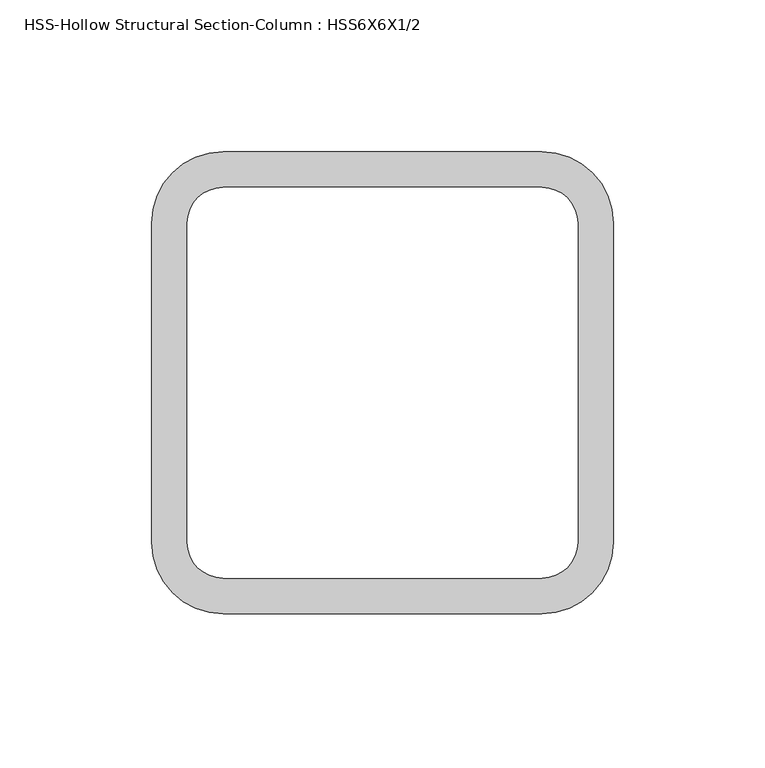
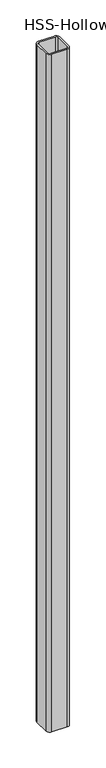
"""IFC4 building model written with IfcOpenShell, lengths in millimetres: column geometry, HSS-Hollow Structural Section-Column : HSS6X6X1/2."""

from ifc_helpers import new_model, si_unit, point, frame, frame_2d, origin, place, context, project, spatial, polyline, circle_curve, trimmed, segment, composite_curve, outline, extrude, source, transform, mapped, element, save


def hss_hollow_structural_section_column_hss6x6x1_2_837c8040(model_context):
    return source(origin(), model_context, "Body", "SweptSolid", [
        extrude(outline(composite_curve([segment(trimmed(circle_curve(frame_2d((52.578, 52.578)), 23.622), [point((52.578, 76.2))], [point((76.2, 52.578))], False, "CARTESIAN"), True, "CONTINUOUS"), segment(polyline([(76.2, 52.578), (76.2, -52.578)]), True, "CONTINUOUS"), segment(trimmed(circle_curve(frame_2d((52.578, -52.578)), 23.622), [point((76.2, -52.578))], [point((52.578, -76.2))], False, "CARTESIAN"), True, "CONTINUOUS"), segment(polyline([(52.578, -76.2), (-52.578, -76.2)]), True, "CONTINUOUS"), segment(trimmed(circle_curve(frame_2d((-52.578, -52.578)), 23.622), [point((-52.578, -76.2))], [point((-76.2, -52.578))], False, "CARTESIAN"), True, "CONTINUOUS"), segment(polyline([(-76.2, -52.578), (-76.2, 52.578)]), True, "CONTINUOUS"), segment(trimmed(circle_curve(frame_2d((-52.578, 52.578)), 23.622), [point((-76.2, 52.578))], [point((-52.578, 76.2))], False, "CARTESIAN"), True, "CONTINUOUS"), segment(polyline([(-52.578, 76.2), (52.578, 76.2)]), True, "CONTINUOUS")], self_intersect=False), holes=[composite_curve([segment(polyline([(52.578, 64.389), (-52.578, 64.389)]), True, "CONTINUOUS"), segment(trimmed(circle_curve(frame_2d((-52.578, 52.578)), 11.811), [point((-52.578, 64.389))], [point((-64.389, 52.578))], True, "CARTESIAN"), True, "CONTINUOUS"), segment(polyline([(-64.389, 52.578), (-64.389, -52.578)]), True, "CONTINUOUS"), segment(trimmed(circle_curve(frame_2d((-52.578, -52.578)), 11.811), [point((-64.389, -52.578))], [point((-52.578, -64.389))], True, "CARTESIAN"), True, "CONTINUOUS"), segment(polyline([(-52.578, -64.389), (52.578, -64.389)]), True, "CONTINUOUS"), segment(trimmed(circle_curve(frame_2d((52.578, -52.578)), 11.811), [point((52.578, -64.389))], [point((64.389, -52.578))], True, "CARTESIAN"), True, "CONTINUOUS"), segment(polyline([(64.389, -52.578), (64.389, 52.578)]), True, "CONTINUOUS"), segment(trimmed(circle_curve(frame_2d((52.578, 52.578)), 11.811), [point((64.389, 52.578))], [point((52.578, 64.389))], True, "CARTESIAN"), True, "CONTINUOUS")], self_intersect=False)]), frame((0.0, 0.0, -609.6), z_axis=(0.0, 0.0, 1.0), x_axis=(1.0, 0.0, 0.0)), (0.0, 0.0, 1.0), 4775.2),
    ])


if __name__ == "__main__":
    model = new_model("IFC4")
    model_context = context("Model", 3, world=origin())
    ifc_project = project(units=[si_unit("LENGTHUNIT", "METRE", prefix="MILLI")], contexts=[model_context])
    site = spatial("IfcSite", under=ifc_project)
    building = spatial("IfcBuilding", under=site)
    placement = place(None, origin())
    hss_hollow_structural_section_column_hss6x6x1_2_shape = hss_hollow_structural_section_column_hss6x6x1_2_837c8040(model_context)
    element("IfcColumn", 1, ObjectType="HSS-Hollow Structural Section-Column : HSS6X6X1/2", at=placement, inside=building, context=model_context, shape_type="MappedRepresentation", body=[
        mapped(hss_hollow_structural_section_column_hss6x6x1_2_shape, transform((0.0, 0.0, 0.0), x_axis=(1.0, 0.0, 0.0), y_axis=(0.0, 1.0, 0.0), z_axis=(0.0, 0.0, 1.0))),
    ])
    save(model, "model.ifc")

# Revit data of these elements
# Type "HSS-Hollow Structural Section-Column : HSS6X6X1/2"
#   Assembly Code = "B10"
#   Shape = "Square"
#   W = 35.1
#   Ht = 0' - 6"
#   b = 0' - 6"
#   kr = 0' - 0.93"
#   t = 0' - 0.465"
#   A = 0.0676389 SF
#   Structural Material [instance default] = Steel ASTM A500, Grade B, Rectangular and Square
# Element 1 (IfcColumn, "HSS-Hollow Structural Section-Column : HSS6X6X1/2")
#   Materials on its faces: "Steel ASTM A500, Grade B, Rectangular and Square"
# Materials
#   "Steel ASTM A500, Grade B, Rectangular and Square": class "Metal", colour RGB 199 199 199, transparency 0, Description = "Carbon steel", Cost = 0
